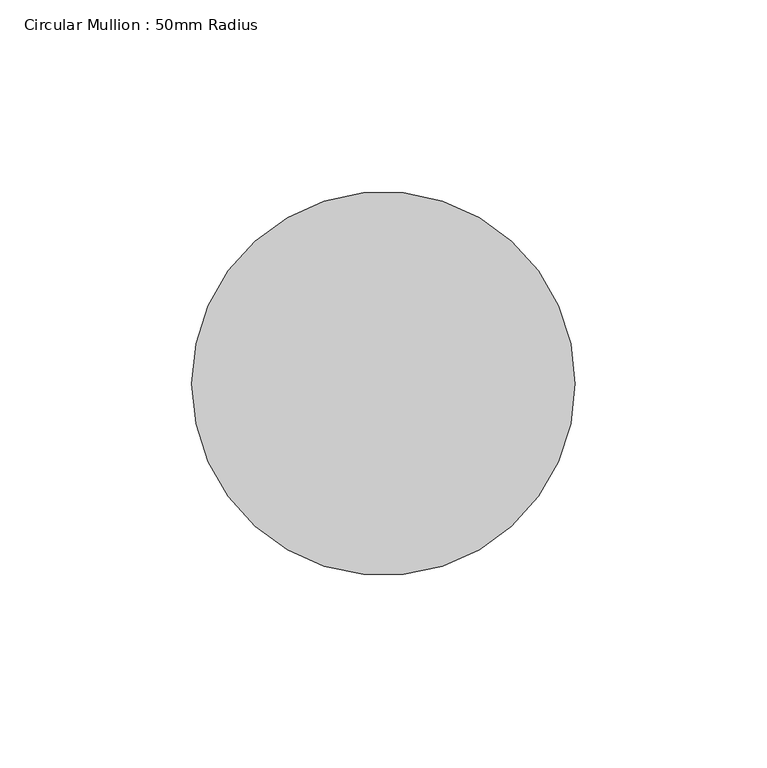
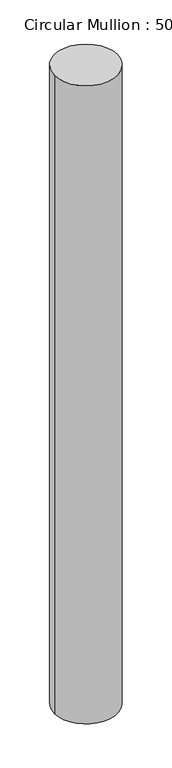
"""IFC4 building model written with IfcOpenShell, lengths in millimetres: member geometry, Circular Mullion : 50mm Radius."""

import ifcopenshell
import ifcopenshell.guid

model = None  # the IFC model being written
_history = None  # IfcOwnerHistory: only IFC2X3 demands one
_inside = {}  # id of a spatial element -> (the spatial element, [elements in it])
_under = {}  # id of a project, library or spatial element -> (it, [spatial elements below it])
_declared = {}  # id of a project -> (the project, [libraries it declares])
_typed = {}  # id of a type object -> (the type object, [elements of that type])
_made_of = {}  # id of a material, layer set ... -> (it, [elements and type objects made of it])


def new_model(schema):
    """Start an empty IFC model of exactly this schema.

    Asked for "IFC4X3", IfcOpenShell would pick the latest addendum, in which some entities
    have other attributes; the version numbers below select the first issue.
    IFC2X3 requires an IfcOwnerHistory on every rooted entity: one is made here for all.
    """
    global model, _history
    if schema == "IFC4X3":
        model = ifcopenshell.file(schema_version=(4, 3, 0, 0))
    else:
        model = ifcopenshell.file(schema=schema)
    _inside.clear()
    _under.clear()
    _declared.clear()
    _typed.clear()
    _made_of.clear()
    _history = None
    if model.schema == "IFC2X3":
        org = make("IfcOrganization", Name="unknown")
        user = make(
            "IfcPersonAndOrganization",
            ThePerson=make("IfcPerson", FamilyName="unknown"),
            TheOrganization=org,
        )
        app = make(
            "IfcApplication",
            ApplicationDeveloper=org,
            Version="unknown",
            ApplicationFullName="unknown",
            ApplicationIdentifier="unknown",
        )
        _history = make(
            "IfcOwnerHistory",
            OwningUser=user,
            OwningApplication=app,
            ChangeAction="ADDED",
            CreationDate=0,
        )
    return model


def make(cls, **values):
    """One entity of the class cls with the attributes given. An attribute that is None is left unset."""
    return model.create_entity(
        cls, **{name: value for name, value in values.items() if value is not None}
    )


def rooted(cls, **values):
    """An entity with a GlobalId (a new one), such as an element, a storey or a relation."""
    return make(cls, GlobalId=ifcopenshell.guid.new(), OwnerHistory=_history, **values)


def si_unit(unit_type, name, prefix=None):
    """IfcSIUnit, for example si_unit("LENGTHUNIT", "METRE", prefix="MILLI")."""
    return make("IfcSIUnit", UnitType=unit_type, Prefix=prefix, Name=name)


def assignment(units):
    """IfcUnitAssignment: the units of a project."""
    return None if units is None else make("IfcUnitAssignment", Units=units)


def point(xyz):
    """IfcCartesianPoint."""
    return None if xyz is None else make("IfcCartesianPoint", Coordinates=xyz)


def direction(xyz):
    """IfcDirection."""
    return None if xyz is None else make("IfcDirection", DirectionRatios=xyz)


def frame(location, z_axis=None, x_axis=None):
    """IfcAxis2Placement3D, a coordinate frame: its origin and axes. An axis left out is left unset."""
    return make(
        "IfcAxis2Placement3D",
        Location=point(location),
        Axis=direction(z_axis),
        RefDirection=direction(x_axis),
    )


def frame_2d(location, x_axis=None):
    """IfcAxis2Placement2D, a coordinate frame in the plane: its origin and x axis."""
    return make(
        "IfcAxis2Placement2D", Location=point(location), RefDirection=direction(x_axis)
    )


def origin():
    """The frame at (0, 0, 0) with its axes left unset."""
    return frame((0.0, 0.0, 0.0))


def origin_2d():
    """The frame at (0, 0) in the plane with its x axis left unset."""
    return frame_2d((0.0, 0.0))


def place(relative_to, where):
    """IfcLocalPlacement: puts the frame where relative to a parent placement (None: the world)."""
    return make(
        "IfcLocalPlacement", PlacementRelTo=relative_to, RelativePlacement=where
    )


def context(
    kind, dimensions, precision=None, world=None, true_north=None, identifier=None
):
    """IfcGeometricRepresentationContext, for example the 3D "Model" context."""
    return make(
        "IfcGeometricRepresentationContext",
        ContextIdentifier=identifier,
        ContextType=kind,
        CoordinateSpaceDimension=dimensions,
        Precision=precision,
        WorldCoordinateSystem=world,
        TrueNorth=true_north,
    )


def project(units=None, contexts=None):
    """IfcProject with its units and contexts."""
    return rooted(
        "IfcProject",
        Name="project",
        RepresentationContexts=contexts,
        UnitsInContext=assignment(units),
    )


def spatial(cls, under=None, at=None, **own):
    """A site, building, storey or space (cls), placed at a placement, below another one or the project."""
    s = rooted(cls, ObjectPlacement=at, **own)
    if under is not None:
        _under.setdefault(under.id(), (under, []))[1].append(s)
    return s


def circle_curve(where, radius):
    """IfcCircle in the frame where."""
    return make("IfcCircle", Position=where, Radius=radius)


def trimmed(basis, trim1, trim2, sense, master):
    """IfcTrimmedCurve: the piece of a basis curve between two trims."""
    return make(
        "IfcTrimmedCurve",
        BasisCurve=basis,
        Trim1=trim1,
        Trim2=trim2,
        SenseAgreement=sense,
        MasterRepresentation=master,
    )


def segment(curve, same_sense, transition):
    """IfcCompositeCurveSegment."""
    return make(
        "IfcCompositeCurveSegment",
        Transition=transition,
        SameSense=same_sense,
        ParentCurve=curve,
    )


def composite_curve(segments, self_intersect=None):
    """IfcCompositeCurve: segments joined end to end."""
    return make("IfcCompositeCurve", Segments=segments, SelfIntersect=self_intersect)


def outline(outer, holes=None, kind="AREA"):
    """IfcArbitraryClosedProfileDef: a profile drawn as a closed curve; with holes, ...WithVoids."""
    if holes is None:
        return make("IfcArbitraryClosedProfileDef", ProfileType=kind, OuterCurve=outer)
    return make(
        "IfcArbitraryProfileDefWithVoids",
        ProfileType=kind,
        OuterCurve=outer,
        InnerCurves=holes,
    )


def extrude(swept, where, along, depth):
    """IfcExtrudedAreaSolid: the profile swept, set in the frame where, extruded along a direction by depth."""
    return make(
        "IfcExtrudedAreaSolid",
        SweptArea=swept,
        Position=where,
        ExtrudedDirection=direction(along),
        Depth=depth,
    )


def shape(context_of_items, identifier, shape_type, items):
    """IfcShapeRepresentation: the items that make up one representation, for example the "Body"."""
    return make(
        "IfcShapeRepresentation",
        ContextOfItems=context_of_items,
        RepresentationIdentifier=identifier,
        RepresentationType=shape_type,
        Items=items,
    )


def source(mapping_origin, context_of_items, identifier, shape_type, items):
    """IfcRepresentationMap: a shape defined once, which mapped items show again and again."""
    return make(
        "IfcRepresentationMap",
        MappingOrigin=mapping_origin,
        MappedRepresentation=shape(context_of_items, identifier, shape_type, items),
    )


def transform(
    local_origin,
    x_axis=None,
    y_axis=None,
    z_axis=None,
    scale=None,
    scale2=None,
    scale3=None,
    uniform=True,
):
    """IfcCartesianTransformationOperator3D, or its non-uniform kind. x_axis, y_axis, z_axis: its Axis1, 2, 3."""
    if uniform:
        return make(
            "IfcCartesianTransformationOperator3D",
            Axis1=direction(x_axis),
            Axis2=direction(y_axis),
            LocalOrigin=point(local_origin),
            Scale=scale,
            Axis3=direction(z_axis),
        )
    return make(
        "IfcCartesianTransformationOperator3DnonUniform",
        Axis1=direction(x_axis),
        Axis2=direction(y_axis),
        LocalOrigin=point(local_origin),
        Scale=scale,
        Axis3=direction(z_axis),
        Scale2=scale2,
        Scale3=scale3,
    )


def mapped(mapping_source, mapping_target):
    """IfcMappedItem: shows the shape of a source again, moved by a transform."""
    return make(
        "IfcMappedItem", MappingSource=mapping_source, MappingTarget=mapping_target
    )


def made_of(thing, what):
    """Note that an element or type object is made of a material, layer set ...; save() writes the relation."""
    if what is not None:
        _made_of.setdefault(what.id(), (what, []))[1].append(thing)
    return thing


def element(
    cls,
    number,
    at=None,
    inside=None,
    cuts=None,
    type_object=None,
    material=None,
    context=None,
    identifier="Body",
    shape_type=None,
    held_by="IfcProductDefinitionShape",
    body=None,
    shapes=None,
    **own,
):
    """One element of the class cls, such as IfcWall. Its Tag is "e" and its number.

    at: its placement. inside: the storey or other place that contains it. cuts: it is an
    opening in that element (IfcRelVoidsElement). A single representation is given by context,
    identifier, shape_type and body (its items); several are given by shapes. held_by: the class
    of the entity that holds the representations. save() writes the other relations.
    """
    e = rooted(cls, Tag="e%d" % number, ObjectPlacement=at, **own)
    if body is not None:
        shapes = [shape(context, identifier, shape_type, body)]
    if shapes is not None:
        e.Representation = make(held_by, Representations=shapes)
    if inside is not None:
        _inside.setdefault(inside.id(), (inside, []))[1].append(e)
    if cuts is not None:
        rooted(
            "IfcRelVoidsElement", RelatingBuildingElement=cuts, RelatedOpeningElement=e
        )
    if type_object is not None:
        _typed.setdefault(type_object.id(), (type_object, []))[1].append(e)
    return made_of(e, material)


def aggregate(whole, parts):
    """IfcRelAggregates: a whole, such as a stair, and the parts it consists of."""
    return rooted("IfcRelAggregates", RelatingObject=whole, RelatedObjects=parts)


def save(model, path):
    """Write the relations noted so far, then the file.

    IfcRelAggregates (storeys below a building ...), IfcRelContainedInSpatialStructure (elements
    in a storey), IfcRelDefinesByType, IfcRelAssociatesMaterial and IfcRelDeclares: one each for
    every whole, place, type object, material and project.
    """
    for whole, parts in _under.values():
        aggregate(whole, parts)
    for where, things in _inside.values():
        rooted(
            "IfcRelContainedInSpatialStructure",
            RelatedElements=things,
            RelatingStructure=where,
        )
    for kind, things in _typed.values():
        rooted("IfcRelDefinesByType", RelatedObjects=things, RelatingType=kind)
    for what, things in _made_of.values():
        rooted("IfcRelAssociatesMaterial", RelatedObjects=things, RelatingMaterial=what)
    for by, libraries in _declared.values():
        rooted("IfcRelDeclares", RelatingContext=by, RelatedDefinitions=libraries)
    model.write(path)


def circular_mullion_50mm_radius_61317bbd(model_context):
    return source(origin(), model_context, "Body", "SweptSolid", [
        extrude(outline(composite_curve([segment(trimmed(circle_curve(origin_2d(), 50.0), [point((50.0, 0.0))], [point((-50.0, 0.0))], False, "CARTESIAN"), True, "CONTINUOUS"), segment(trimmed(circle_curve(origin_2d(), 50.0), [point((-50.0, 0.0))], [point((50.0, 0.0))], False, "CARTESIAN"), True, "CONTINUOUS")], self_intersect=False)), frame((0.0, 0.0, -1069.7089872), z_axis=(0.0, 0.0, 1.0), x_axis=(1.0, 0.0, 0.0)), (0.0, 0.0, 1.0), 1069.7089872),
    ])


if __name__ == "__main__":
    model = new_model("IFC4")
    model_context = context("Model", 3, world=origin())
    ifc_project = project(units=[si_unit("LENGTHUNIT", "METRE", prefix="MILLI")], contexts=[model_context])
    site = spatial("IfcSite", under=ifc_project)
    building = spatial("IfcBuilding", under=site)
    placement = place(None, origin())
    circular_mullion_50mm_radius_shape = circular_mullion_50mm_radius_61317bbd(model_context)
    element("IfcMember", 1, ObjectType="Circular Mullion : 50mm Radius", at=placement, inside=building, context=model_context, shape_type="MappedRepresentation", body=[
        mapped(circular_mullion_50mm_radius_shape, transform((0.0, 0.0, 0.0), x_axis=(1.0, 0.0, 0.0), y_axis=(0.0, 1.0, 0.0), z_axis=(0.0, 0.0, 1.0))),
    ])
    save(model, "model.ifc")

# Revit data of these elements
# Type "Circular Mullion : 50mm Radius"
#   built-in parameter 1007350 = 0.164042 (stored number, unit not read)
# Element 1 (IfcMember, "Circular Mullion : 50mm Radius")
#   Materials on its faces: "Aluminium"
# Materials
#   "Aluminium": class "Metal", colour RGB 247 247 247, transparency 0, Description = "Aluminium 6061", Cost = 0
